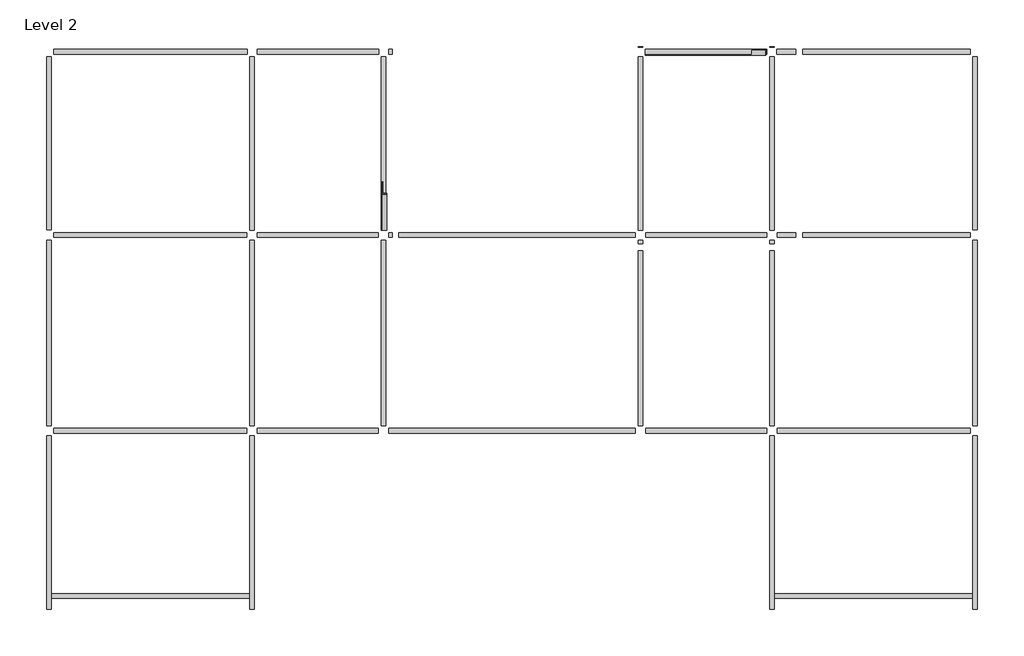
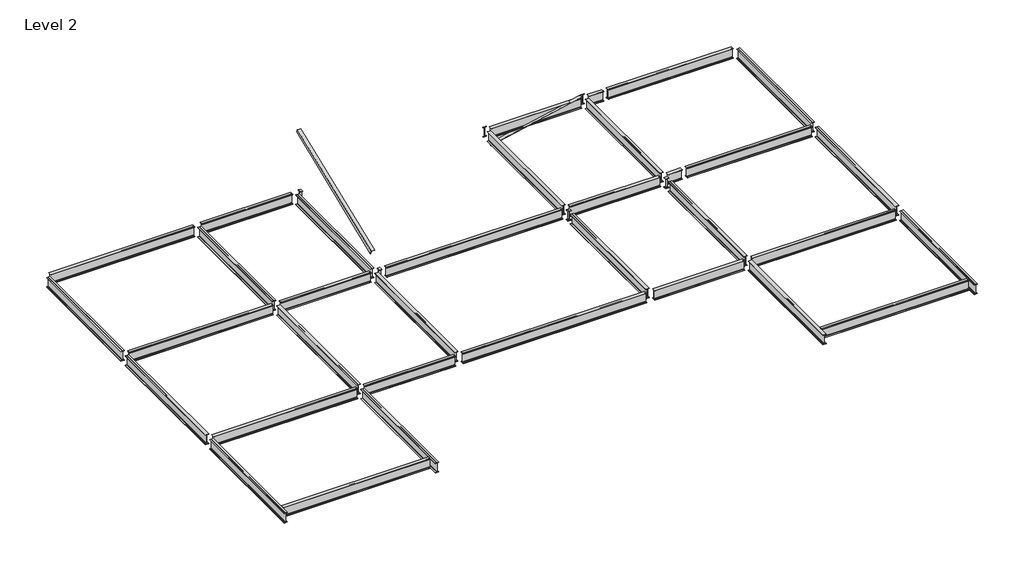
# One storey: 40 beams, 2 members.
# Revit data of these elements (continued)
# Type "W-Wide Flange2 : W18X40"
#   Assembly Code = "B10"
#   W = 40
#   Length [instance default] = 5' - 0"
#   bf = 0' - 6.02"
#   d = 1' - 5.9"
#   k = 0' - 1 3/16"
#   k2 = 0' - 0.6625"
#   tf = 0' - 0.525"
#   tw = 0' - 0.315"
#   A = 0.0819444 SF
#   Structural Material [instance default] = Steel ASTM A992
# Type "L-Angle2 : L6X6X3/8"
#   Assembly Code = "B10"
#   k = 0' - 0 7/8"
#   W = 14.9
#   Length [instance default] = 5' - 0"
#   b = 0' - 6"
#   d = 0' - 6"
#   t = 0' - 0 3/8"
#   x = 0' - 1.62"
#   y = 0' - 1.62"
#   A = 0.0304167 SF
#   Structural Material [instance default] = Steel ASTM A36
# Elements 1, 2, 3, 4, 5, 6, 7, 8, 9, 10, 11, 12, 13, 14, 15, 16, 17, 18, 19, 20, 21, 22, 23, 24, 25, 26, 27, 28, 29, 30, 31, 32, 33, 34, 35, 36, 37, 38, 39, 40 (IfcBeam, "W-Wide Flange2 : W18X40")
#   Structural Material = Steel ASTM A992
#   Phase Created = New Construction
#   Materials on its faces: "Steel ASTM A992"
# Elements 41, 42 (IfcMember, "L-Angle2 : L6X6X3/8")
#   Structural Material = Steel ASTM A36
#   Phase Created = New Construction
#   Materials on its faces: "Steel ASTM A36"
# Materials
#   "Steel ASTM A992": class "Metal", colour RGB 199 199 199, transparency 0, Description = "Structural steel 50ksi", Cost = 0
#   "Steel ASTM A36": class "Metal", colour RGB 199 199 199, transparency 0, Description = "Structural steel, ASTM A36 Grade B, mill finish", Cost = 0
